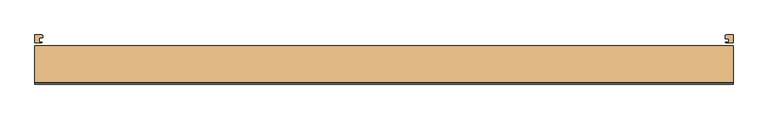
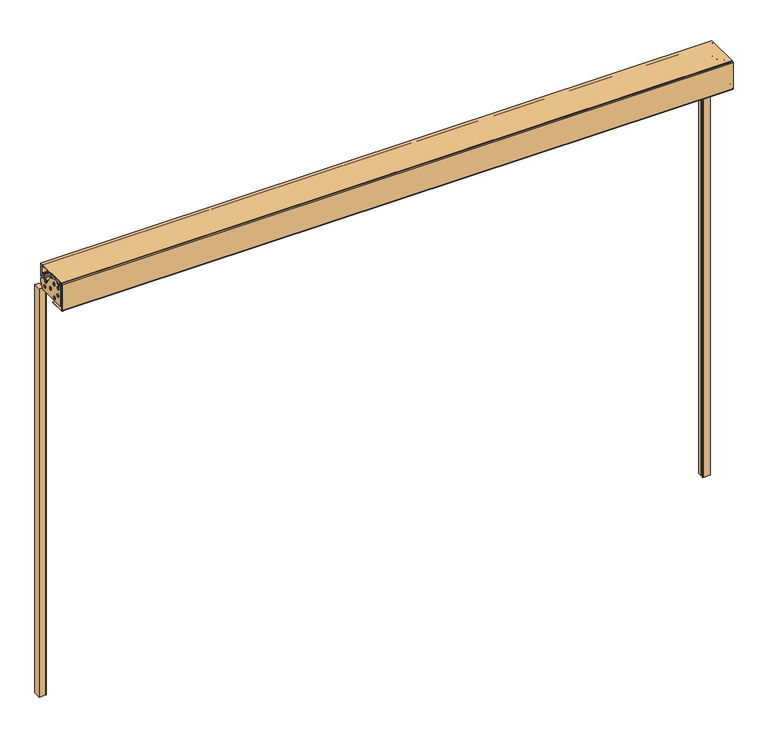
"""IFC4 building model written with IfcOpenShell, lengths in millimetres: door geometry, Otomatik Kapı-Tek Kanat : Otomatik Kapı - Tek Kanat."""

from ifc_helpers import new_model, si_unit, point, frame, frame_2d, origin, origin_with_axes, place, context, project, spatial, polyline, circle_curve, trimmed, segment, composite_curve, outline, extrude, source, transform, mapped, element, save
from ifc_brep_helpers import plane_surface, cylinder_surface, revolved_surface, advanced_brep


def door_4716b48a(model_context):
    return source(origin(), model_context, "Body", "SolidModel", [
        advanced_brep(
        [(1597.0, -299.2542528, 2176.1817261), (1597.0, -285.0832683, 2176.1817261), (1597.0, -280.0474706, 2181.1107692), (1597.0, -280.0474706, 2184.2914876), (1597.0, -239.7553085, 2184.2914876), (1597.0, -239.7553085, 2181.2186799), (1597.0, -234.7183548, 2176.1817261), (1597.0, -226.0109102, 2176.1817261), (1597.0, -221.657188, 2173.7066015), (1597.0, -194.0014824, 2126.1506632), (1597.0, -189.1337497, 2122.4873595), (1597.0, -183.2436236, 2122.4873595), (1597.0, -178.2215661, 2127.509417), (1597.0, -178.2066698, 2136.5727956), (1597.0, -146.96299, 2136.5727956), (1597.0, -146.96299, 2125.3902264), (1597.0, -146.0348324, 2123.5834794), (1597.0, -145.0, 2121.6341872), (1597.0, -145.0, 2108.8285097), (1597.0, -145.5976831, 2106.353385), (1597.0, -161.6461091, 2078.6102552), (1597.0, -165.9998314, 2076.1339745), (1597.0, -299.2542528, 2076.1339745), (1597.0, -304.2900505, 2081.1697722), (1597.0, -304.2900505, 2171.1459284), (1597.0, -252.8153193, 2150.4871347), (1597.0, -252.8153193, 2165.6823884), (1597.0, -286.1075375, 2150.4871347), (1597.0, -286.1075375, 2165.6823884), (1597.0, -284.058999, 2111.9024734), (1597.0, -284.058999, 2126.9266302), (1597.0, -223.621334, 2111.7978536), (1597.0, -223.621334, 2127.0312501), (1597.0, -255.888127, 2083.6460529), (1597.0, -255.888127, 2098.8413066), (1597.0, -176.2436798, 2091.7558144), (1597.0, -176.2436798, 2106.7799712), (1600.0, -299.2542528, 2176.1817261), (1600.0, -304.2900505, 2171.1459284), (1600.0, -304.2900505, 2081.1697722), (1600.0, -299.2542528, 2076.1339745), (1600.0, -165.9998314, 2076.1339745), (1600.0, -161.6461091, 2078.6102552), (1600.0, -145.5976831, 2106.353385), (1600.0, -145.0, 2108.8285097), (1600.0, -145.0, 2121.6341872), (1600.0, -146.0451322, 2123.567749), (1600.0, -146.96299, 2125.3902264), (1600.0, -146.96299, 2136.5727956), (1600.0, -178.2066698, 2136.5727956), (1600.0, -178.2066698, 2127.509417), (1600.0, -183.2436236, 2122.4873595), (1600.0, -189.1337497, 2122.4873595), (1600.0, -194.0014824, 2126.1506632), (1600.0, -221.657188, 2173.7066015), (1600.0, -226.0109102, 2176.1817261), (1600.0, -234.7183548, 2176.1817261), (1600.0, -239.7553085, 2181.2186799), (1600.0, -239.7553085, 2184.2914876), (1600.0, -280.0474706, 2184.2914876), (1600.0, -280.0474706, 2181.1107692), (1600.0, -285.0832683, 2176.1817261), (1600.0, -252.8153193, 2150.4871347), (1600.0, -252.8153193, 2165.6823884), (1600.0, -286.1075375, 2150.4871347), (1600.0, -286.1075375, 2165.6823884), (1600.0, -284.058999, 2111.9024734), (1600.0, -284.058999, 2126.9266302), (1600.0, -223.621334, 2111.7978536), (1600.0, -223.621334, 2127.0312501), (1600.0, -255.888127, 2083.6460529), (1600.0, -255.888127, 2098.8413066), (1600.0, -176.2436798, 2091.7558144), (1600.0, -176.2436798, 2106.7799712)],
        [
            (0, 1),
            (1, 2, circle_curve(frame((1597.0, -285.0832683, 2181.2186799), z_axis=(1.0, 0.0, 0.0), x_axis=(0.0, 0.0, 1.0)), 5.0369538)),
            (2, 3),
            (3, 4),
            (4, 5),
            (5, 6, circle_curve(frame((1597.0, -234.7183548, 2181.2186799), z_axis=(1.0, 0.0, 0.0), x_axis=(0.0, 0.0, 1.0)), 5.0369538)),
            (6, 7),
            (7, 8, circle_curve(frame((1597.0, -225.960249, 2171.2041971), z_axis=(-1.0, 0.0, 0.0), x_axis=(0.0, 0.0, 1.0)), 4.9777868)),
            (8, 9),
            (9, 10, circle_curve(frame((1597.0, -189.1337497, 2127.5530897), z_axis=(1.0, 0.0, 0.0), x_axis=(0.0, 0.0, 1.0)), 5.0657302)),
            (10, 11),
            (11, 12, circle_curve(frame((1597.0, -183.2436236, 2127.509417), z_axis=(1.0, 0.0, 0.0), x_axis=(0.0, 0.0, 1.0)), 5.0220574)),
            (12, 13),
            (13, 14),
            (14, 15),
            (15, 16, circle_curve(frame((1597.0, -144.9082992, 2125.3039782), z_axis=(1.0, 0.0, 0.0), x_axis=(0.0, 0.0, 1.0)), 2.0565002)),
            (16, 17, circle_curve(frame((1597.0, -147.3111729, 2121.6341872), z_axis=(-1.0, 0.0, 0.0), x_axis=(0.0, 0.0, 1.0)), 2.3111729)),
            (17, 18),
            (18, 19, circle_curve(frame((1597.0, -149.4842362, 2108.6016195), z_axis=(-1.0, 0.0, 0.0), x_axis=(0.0, 0.0, 1.0)), 4.4899725)),
            (19, 20),
            (20, 21, circle_curve(frame((1597.0, -165.9399214, 2081.0940748), z_axis=(-1.0, 0.0, 0.0), x_axis=(0.0, 0.0, 1.0)), 4.9604621)),
            (21, 22),
            (22, 23, circle_curve(frame((1597.0, -299.2542528, 2081.1697722), z_axis=(-1.0, 0.0, 0.0), x_axis=(0.0, 0.0, 1.0)), 5.0357977)),
            (23, 24),
            (24, 0, circle_curve(frame((1597.0, -299.2542528, 2171.1459284), z_axis=(-1.0, 0.0, 0.0), x_axis=(0.0, 0.0, 1.0)), 5.0357977)),
            (25, 26, circle_curve(frame((1597.0, -252.8153193, 2158.0847616), z_axis=(1.0, 0.0, 0.0), x_axis=(0.0, 0.0, 1.0)), 7.5976269)),
            (26, 25, circle_curve(frame((1597.0, -252.8153193, 2158.0847616), z_axis=(1.0, 0.0, 0.0), x_axis=(0.0, 0.0, 1.0)), 7.5976269)),
            (27, 28, circle_curve(frame((1597.0, -286.1075375, 2158.0847616), z_axis=(1.0, 0.0, 0.0), x_axis=(0.0, 0.0, 1.0)), 7.5976269)),
            (28, 27, circle_curve(frame((1597.0, -286.1075375, 2158.0847616), z_axis=(1.0, 0.0, 0.0), x_axis=(0.0, 0.0, 1.0)), 7.5976269)),
            (29, 30, circle_curve(frame((1597.0, -284.058999, 2119.4145518), z_axis=(1.0, 0.0, 0.0), x_axis=(0.0, 0.0, 1.0)), 7.5120784)),
            (30, 29, circle_curve(frame((1597.0, -284.058999, 2119.4145518), z_axis=(1.0, 0.0, 0.0), x_axis=(0.0, 0.0, 1.0)), 7.5120784)),
            (31, 32, circle_curve(frame((1597.0, -223.621334, 2119.4145518), z_axis=(1.0, 0.0, 0.0), x_axis=(0.0, 0.0, 1.0)), 7.6166982)),
            (32, 31, circle_curve(frame((1597.0, -223.621334, 2119.4145518), z_axis=(1.0, 0.0, 0.0), x_axis=(0.0, 0.0, 1.0)), 7.6166982)),
            (33, 34, circle_curve(frame((1597.0, -255.888127, 2091.2436798), z_axis=(1.0, 0.0, 0.0), x_axis=(0.0, 0.0, 1.0)), 7.5976269)),
            (34, 33, circle_curve(frame((1597.0, -255.888127, 2091.2436798), z_axis=(1.0, 0.0, 0.0), x_axis=(0.0, 0.0, 1.0)), 7.5976269)),
            (35, 36, circle_curve(frame((1597.0, -176.2436798, 2099.2678928), z_axis=(1.0, 0.0, 0.0), x_axis=(0.0, 0.0, 1.0)), 7.5120784)),
            (36, 35, circle_curve(frame((1597.0, -176.2436798, 2099.2678928), z_axis=(1.0, 0.0, 0.0), x_axis=(0.0, 0.0, 1.0)), 7.5120784)),
            (37, 38, circle_curve(frame((1600.0, -299.2542528, 2171.1459284), z_axis=(1.0, 0.0, 0.0), x_axis=(0.0, 0.0, 1.0)), 5.0357977)),
            (38, 39),
            (39, 40, circle_curve(frame((1600.0, -299.2542528, 2081.1697722), z_axis=(1.0, 0.0, 0.0), x_axis=(0.0, 0.0, 1.0)), 5.0357977)),
            (40, 41),
            (41, 42, circle_curve(frame((1600.0, -165.9399214, 2081.0940748), z_axis=(1.0, 0.0, 0.0), x_axis=(0.0, 0.0, 1.0)), 4.9604621)),
            (42, 43),
            (43, 44, circle_curve(frame((1600.0, -149.4842362, 2108.6016195), z_axis=(1.0, 0.0, 0.0), x_axis=(0.0, 0.0, 1.0)), 4.4899725)),
            (44, 45),
            (45, 46, circle_curve(frame((1600.0, -147.3111729, 2121.6341872), z_axis=(1.0, 0.0, 0.0), x_axis=(0.0, 0.0, 1.0)), 2.3111729)),
            (46, 47, circle_curve(frame((1600.0, -144.9082992, 2125.3039782), z_axis=(-1.0, 0.0, 0.0), x_axis=(0.0, 0.0, 1.0)), 2.0565002)),
            (47, 48),
            (48, 49),
            (49, 50),
            (50, 51, circle_curve(frame((1600.0, -183.2436236, 2127.509417), z_axis=(-1.0, 0.0, 0.0), x_axis=(0.0, 0.0, 1.0)), 5.0220574)),
            (51, 52),
            (52, 53, circle_curve(frame((1600.0, -189.1337497, 2127.5530897), z_axis=(-1.0, 0.0, 0.0), x_axis=(0.0, 0.0, 1.0)), 5.0657302)),
            (53, 54),
            (54, 55, circle_curve(frame((1600.0, -225.960249, 2171.2041971), z_axis=(1.0, 0.0, 0.0), x_axis=(0.0, 0.0, 1.0)), 4.9777868)),
            (55, 56),
            (56, 57, circle_curve(frame((1600.0, -234.7183548, 2181.2186799), z_axis=(-1.0, 0.0, 0.0), x_axis=(0.0, 0.0, 1.0)), 5.0369538)),
            (57, 58),
            (58, 59),
            (59, 60),
            (60, 61, circle_curve(frame((1600.0, -285.0832683, 2181.2186799), z_axis=(-1.0, 0.0, 0.0), x_axis=(0.0, 0.0, 1.0)), 5.0369538)),
            (61, 37),
            (62, 63, circle_curve(frame((1600.0, -252.8153193, 2158.0847616), z_axis=(-1.0, 0.0, 0.0), x_axis=(0.0, 0.0, 1.0)), 7.5976269)),
            (63, 62, circle_curve(frame((1600.0, -252.8153193, 2158.0847616), z_axis=(-1.0, 0.0, 0.0), x_axis=(0.0, 0.0, 1.0)), 7.5976269)),
            (64, 65, circle_curve(frame((1600.0, -286.1075375, 2158.0847616), z_axis=(-1.0, 0.0, 0.0), x_axis=(0.0, 0.0, 1.0)), 7.5976269)),
            (65, 64, circle_curve(frame((1600.0, -286.1075375, 2158.0847616), z_axis=(-1.0, 0.0, 0.0), x_axis=(0.0, 0.0, 1.0)), 7.5976269)),
            (66, 67, circle_curve(frame((1600.0, -284.058999, 2119.4145518), z_axis=(-1.0, 0.0, 0.0), x_axis=(0.0, 0.0, 1.0)), 7.5120784)),
            (67, 66, circle_curve(frame((1600.0, -284.058999, 2119.4145518), z_axis=(-1.0, 0.0, 0.0), x_axis=(0.0, 0.0, 1.0)), 7.5120784)),
            (68, 69, circle_curve(frame((1600.0, -223.621334, 2119.4145518), z_axis=(-1.0, 0.0, 0.0), x_axis=(0.0, 0.0, 1.0)), 7.6166982)),
            (69, 68, circle_curve(frame((1600.0, -223.621334, 2119.4145518), z_axis=(-1.0, 0.0, 0.0), x_axis=(0.0, 0.0, 1.0)), 7.6166982)),
            (70, 71, circle_curve(frame((1600.0, -255.888127, 2091.2436798), z_axis=(-1.0, 0.0, 0.0), x_axis=(0.0, 0.0, 1.0)), 7.5976269)),
            (71, 70, circle_curve(frame((1600.0, -255.888127, 2091.2436798), z_axis=(-1.0, 0.0, 0.0), x_axis=(0.0, 0.0, 1.0)), 7.5976269)),
            (72, 73, circle_curve(frame((1600.0, -176.2436798, 2099.2678928), z_axis=(-1.0, 0.0, 0.0), x_axis=(0.0, 0.0, 1.0)), 7.5120784)),
            (73, 72, circle_curve(frame((1600.0, -176.2436798, 2099.2678928), z_axis=(-1.0, 0.0, 0.0), x_axis=(0.0, 0.0, 1.0)), 7.5120784)),
            (0, 37),
            (61, 1),
            (60, 2),
            (59, 3),
            (58, 4),
            (57, 5),
            (56, 6),
            (55, 7),
            (54, 8),
            (53, 9),
            (52, 10),
            (51, 11),
            (50, 12),
            (49, 13),
            (48, 14),
            (47, 15),
            (46, 16),
            (45, 17),
            (44, 18),
            (43, 19),
            (42, 20),
            (41, 21),
            (40, 22),
            (39, 23),
            (38, 24),
            (25, 62),
            (63, 26),
            (27, 64),
            (65, 28),
            (29, 66),
            (67, 30),
            (31, 68),
            (69, 32),
            (33, 70),
            (71, 34),
            (35, 72),
            (73, 36),
        ],
        [
            plane_surface(frame((1597.0, -145.0, 2060.0), z_axis=(-1.0, 0.0, 0.0), x_axis=(0.0, -1.0, 0.0))),
            plane_surface(frame((1600.0, -145.0, 2060.0), z_axis=(1.0, 0.0, 0.0), x_axis=(0.0, -1.0, 0.0))),
            plane_surface(frame((1597.0, -299.2542528, 2176.1817261), z_axis=(0.0, 0.0, 1.0), x_axis=(1.0, 0.0, 0.0))),
            revolved_surface(polyline([(1600.0, -285.0832683, 2186.2556337), (1597.0, -285.0832683, 2186.2556337)]), (1597.0, -285.0832683, 2181.2186799), (1.0, 0.0, 0.0)),
            plane_surface(frame((1597.0, -280.0474706, 2181.1107692), z_axis=(0.0, -1.0, 0.0), x_axis=(1.0, 0.0, 0.0))),
            plane_surface(frame((1597.0, -280.0474706, 2184.2914876), z_axis=(0.0, 0.0, 1.0), x_axis=(1.0, 0.0, 0.0))),
            plane_surface(frame((1597.0, -239.7553085, 2184.2914876), z_axis=(0.0, 1.0, 0.0), x_axis=(1.0, 0.0, 0.0))),
            revolved_surface(polyline([(1600.0, -234.7183548, 2186.2556337), (1597.0, -234.7183548, 2186.2556337)]), (1597.0, -234.7183548, 2181.2186799), (1.0, 0.0, 0.0)),
            plane_surface(frame((1597.0, -234.7183548, 2176.1817261), z_axis=(0.0, 0.0, 1.0), x_axis=(1.0, 0.0, 0.0))),
            cylinder_surface(frame((1597.0, -225.960249, 2171.2041971), z_axis=(-1.0, 0.0, 0.0), x_axis=(0.0, 0.0, 1.0)), 4.9777868),
            plane_surface(frame((1597.0, -221.657188, 2173.7066015), z_axis=(0.0, 0.8644526484288484, 0.5027142514633436), x_axis=(1.0, 0.0, 0.0))),
            revolved_surface(polyline([(1600.0, -189.1337497, 2132.6188199), (1597.0, -189.1337497, 2132.6188199)]), (1597.0, -189.1337497, 2127.5530897), (1.0, 0.0, 0.0)),
            plane_surface(frame((1597.0, -189.1337497, 2122.4873595), z_axis=(0.0, 0.0, 1.0), x_axis=(1.0, 0.0, 0.0))),
            revolved_surface(polyline([(1600.0, -183.2436236, 2132.5314744), (1597.0, -183.2436236, 2132.5314744)]), (1597.0, -183.2436236, 2127.509417), (1.0, 0.0, 0.0)),
            plane_surface(frame((1597.0, -178.2066698, 2127.509417), z_axis=(0.0, -1.0, 0.0), x_axis=(1.0, 0.0, 0.0))),
            plane_surface(frame((1597.0, -178.2066698, 2136.5727956), z_axis=(0.0, 0.0, 1.0), x_axis=(1.0, 0.0, 0.0))),
            plane_surface(frame((1597.0, -146.96299, 2136.5727956), z_axis=(0.0, 1.0, 0.0), x_axis=(1.0, 0.0, 0.0))),
            revolved_surface(polyline([(1600.0, -144.9082992, 2127.3604784), (1597.0, -144.9082992, 2127.3604784)]), (1597.0, -144.9082992, 2125.3039782), (1.0, 0.0, 0.0)),
            cylinder_surface(frame((1597.0, -147.3111729, 2121.6341872), z_axis=(-1.0, 0.0, 0.0), x_axis=(0.0, 0.0, 1.0)), 2.3111729),
            plane_surface(frame((1597.0, -145.0, 2121.6341872), z_axis=(0.0, 1.0, 0.0), x_axis=(1.0, 0.0, 0.0))),
            cylinder_surface(frame((1597.0, -149.4842362, 2108.6016195), z_axis=(-1.0, 0.0, 0.0), x_axis=(0.0, 0.0, 1.0)), 4.4899725),
            plane_surface(frame((1597.0, -145.5976831, 2106.353385), z_axis=(0.0, 0.8656073271784467, -0.5007234317814432), x_axis=(1.0, 0.0, 0.0))),
            cylinder_surface(frame((1597.0, -165.9399214, 2081.0940748), z_axis=(-1.0, 0.0, 0.0), x_axis=(0.0, 0.0, 1.0)), 4.9604621),
            plane_surface(frame((1597.0, -165.9998314, 2076.1339745), z_axis=(0.0, 0.0, -1.0), x_axis=(1.0, 0.0, 0.0))),
            cylinder_surface(frame((1597.0, -299.2542528, 2081.1697722), z_axis=(-1.0, 0.0, 0.0), x_axis=(0.0, 0.0, 1.0)), 5.0357977),
            plane_surface(frame((1597.0, -304.2900505, 2081.1697722), z_axis=(0.0, -1.0, 0.0), x_axis=(1.0, 0.0, 0.0))),
            cylinder_surface(frame((1597.0, -299.2542528, 2171.1459284), z_axis=(-1.0, 0.0, 0.0), x_axis=(0.0, 0.0, 1.0)), 5.0357977),
            revolved_surface(polyline([(1600.0, -252.8153193, 2165.6823885), (1597.0, -252.8153193, 2165.6823885)]), (1597.0, -252.8153193, 2158.0847616), (1.0, 0.0, 0.0)),
            revolved_surface(polyline([(1600.0, -286.1075375, 2165.6823885), (1597.0, -286.1075375, 2165.6823885)]), (1597.0, -286.1075375, 2158.0847616), (1.0, 0.0, 0.0)),
            revolved_surface(polyline([(1600.0, -284.058999, 2126.9266302), (1597.0, -284.058999, 2126.9266302)]), (1597.0, -284.058999, 2119.4145518), (1.0, 0.0, 0.0)),
            revolved_surface(polyline([(1600.0, -223.621334, 2127.03125), (1597.0, -223.621334, 2127.03125)]), (1597.0, -223.621334, 2119.4145518), (1.0, 0.0, 0.0)),
            revolved_surface(polyline([(1600.0, -255.888127, 2098.8413066999997), (1597.0, -255.888127, 2098.8413066999997)]), (1597.0, -255.888127, 2091.2436798), (1.0, 0.0, 0.0)),
            revolved_surface(polyline([(1600.0, -176.2436798, 2106.7799712), (1597.0, -176.2436798, 2106.7799712)]), (1597.0, -176.2436798, 2099.2678928), (1.0, 0.0, 0.0)),
        ],
        [
            (0, [[1, 2, 3, 4, 5, 6, 7, 8, 9, 10, 11, 12, 13, 14, 15, 16, 17, 18, 19, 20, 21, 22, 23, 24, 25], [26, 27], [28, 29], [30, 31], [32, 33], [34, 35], [36, 37]]),
            (1, [[38, 39, 40, 41, 42, 43, 44, 45, 46, 47, 48, 49, 50, 51, 52, 53, 54, 55, 56, 57, 58, 59, 60, 61, 62], [63, 64], [65, 66], [67, 68], [69, 70], [71, 72], [73, 74]]),
            (2, [[-1, 75, -62, 76]]),
            (3, [[-2, -76, -61, 77]]),
            (4, [[-3, -77, -60, 78]]),
            (5, [[-4, -78, -59, 79]]),
            (6, [[-5, -79, -58, 80]]),
            (7, [[-6, -80, -57, 81]]),
            (8, [[-7, -81, -56, 82]]),
            (9, [[-8, -82, -55, 83]]),
            (10, [[-9, -83, -54, 84]]),
            (11, [[-10, -84, -53, 85]]),
            (12, [[-11, -85, -52, 86]]),
            (13, [[-12, -86, -51, 87]]),
            (14, [[-13, -87, -50, 88]]),
            (15, [[-14, -88, -49, 89]]),
            (16, [[-15, -89, -48, 90]]),
            (17, [[-16, -90, -47, 91]]),
            (18, [[-17, -91, -46, 92]]),
            (19, [[-18, -92, -45, 93]]),
            (20, [[-19, -93, -44, 94]]),
            (21, [[-20, -94, -43, 95]]),
            (22, [[-21, -95, -42, 96]]),
            (23, [[-22, -96, -41, 97]]),
            (24, [[-23, -97, -40, 98]]),
            (25, [[-24, -98, -39, 99]]),
            (26, [[-25, -99, -38, -75]]),
            (27, [[-26, 100, -64, 101]]),
            (27, [[-27, -101, -63, -100]]),
            (28, [[-28, 102, -66, 103]]),
            (28, [[-29, -103, -65, -102]]),
            (29, [[-30, 104, -68, 105]]),
            (29, [[-31, -105, -67, -104]]),
            (30, [[-32, 106, -70, 107]]),
            (30, [[-33, -107, -69, -106]]),
            (31, [[-34, 108, -72, 109]]),
            (31, [[-35, -109, -71, -108]]),
            (32, [[-36, 110, -74, 111]]),
            (32, [[-37, -111, -73, -110]]),
        ],
    ),
        advanced_brep(
        [(-1597.0, -239.7553085, 2184.2914876), (-1597.0, -280.0474706, 2184.2914876), (-1597.0, -280.0474706, 2181.1107692), (-1597.0, -285.0832683, 2176.1817261), (-1597.0, -299.2542528, 2176.1817261), (-1597.0, -304.2900505, 2171.1459284), (-1597.0, -304.2900505, 2081.1697722), (-1597.0, -299.2542528, 2076.1339745), (-1597.0, -165.9998314, 2076.1339745), (-1597.0, -161.6461091, 2078.6102552), (-1597.0, -145.5976831, 2106.353385), (-1597.0, -145.0, 2108.8285097), (-1597.0, -145.0, 2121.6341872), (-1597.0, -146.0451322, 2123.567749), (-1597.0, -146.96299, 2125.3902264), (-1597.0, -146.96299, 2136.5727956), (-1597.0, -178.2066698, 2136.5727956), (-1597.0, -178.2066698, 2127.509417), (-1597.0, -183.2436236, 2122.4873595), (-1597.0, -189.1337497, 2122.4873595), (-1597.0, -194.0014824, 2126.1506632), (-1597.0, -221.657188, 2173.7066015), (-1597.0, -226.0109102, 2176.1817261), (-1597.0, -234.7183548, 2176.1817261), (-1597.0, -239.7553085, 2181.2186799), (-1597.0, -176.2436798, 2106.7799712), (-1597.0, -176.2436798, 2091.7558144), (-1597.0, -223.621334, 2127.0312501), (-1597.0, -223.621334, 2111.7978536), (-1597.0, -252.8153193, 2165.6823884), (-1597.0, -252.8153193, 2150.4871347), (-1597.0, -286.1075375, 2165.6823884), (-1597.0, -286.1075375, 2150.4871347), (-1597.0, -284.058999, 2126.9266302), (-1597.0, -284.058999, 2111.9024734), (-1597.0, -255.888127, 2098.8413066), (-1597.0, -255.888127, 2083.6460529), (-1600.0, -239.7553085, 2184.2914876), (-1600.0, -239.7553085, 2181.2186799), (-1600.0, -234.7183548, 2176.1817261), (-1600.0, -226.0109102, 2176.1817261), (-1600.0, -221.657188, 2173.7066015), (-1600.0, -194.0014824, 2126.1506632), (-1600.0, -189.1337497, 2122.4873595), (-1600.0, -183.2436236, 2122.4873595), (-1600.0, -178.2215661, 2127.509417), (-1600.0, -178.2066698, 2136.5727956), (-1600.0, -146.96299, 2136.5727956), (-1600.0, -146.96299, 2125.3902264), (-1600.0, -146.0348324, 2123.5834794), (-1600.0, -145.0, 2121.6341872), (-1600.0, -145.0, 2108.8285097), (-1600.0, -145.5976831, 2106.353385), (-1600.0, -161.6461091, 2078.6102552), (-1600.0, -165.9998314, 2076.1339745), (-1600.0, -299.2542528, 2076.1339745), (-1600.0, -304.2900505, 2081.1697722), (-1600.0, -304.2900505, 2171.1459284), (-1600.0, -299.2542528, 2176.1817261), (-1600.0, -285.0832683, 2176.1817261), (-1600.0, -280.0474706, 2181.1107692), (-1600.0, -280.0474706, 2184.2914876), (-1600.0, -176.2436798, 2106.7799712), (-1600.0, -176.2436798, 2091.7558144), (-1600.0, -223.621334, 2127.0312501), (-1600.0, -223.621334, 2111.7978536), (-1600.0, -252.8153193, 2165.6823884), (-1600.0, -252.8153193, 2150.4871347), (-1600.0, -286.1075375, 2165.6823884), (-1600.0, -286.1075375, 2150.4871347), (-1600.0, -284.058999, 2126.9266302), (-1600.0, -284.058999, 2111.9024734), (-1600.0, -255.888127, 2098.8413066), (-1600.0, -255.888127, 2083.6460529)],
        [
            (0, 1),
            (1, 2),
            (2, 3, circle_curve(frame((-1597.0, -285.0832683, 2181.2186799), z_axis=(-1.0, 0.0, 0.0), x_axis=(0.0, 0.0, -1.0)), 5.0369538)),
            (3, 4),
            (4, 5, circle_curve(frame((-1597.0, -299.2542528, 2171.1459284), z_axis=(1.0, 0.0, 0.0), x_axis=(0.0, 0.0, -1.0)), 5.0357977)),
            (5, 6),
            (6, 7, circle_curve(frame((-1597.0, -299.2542528, 2081.1697722), z_axis=(1.0, 0.0, 0.0), x_axis=(0.0, 0.0, -1.0)), 5.0357977)),
            (7, 8),
            (8, 9, circle_curve(frame((-1597.0, -165.9399214, 2081.0940748), z_axis=(1.0, 0.0, 0.0), x_axis=(0.0, 0.0, -1.0)), 4.9604621)),
            (9, 10),
            (10, 11, circle_curve(frame((-1597.0, -149.4842362, 2108.6016195), z_axis=(1.0, 0.0, 0.0), x_axis=(0.0, 0.0, -1.0)), 4.4899725)),
            (11, 12),
            (12, 13, circle_curve(frame((-1597.0, -147.3111729, 2121.6341872), z_axis=(1.0, 0.0, 0.0), x_axis=(0.0, 0.0, -1.0)), 2.3111729)),
            (13, 14, circle_curve(frame((-1597.0, -144.9082992, 2125.3039782), z_axis=(-1.0, 0.0, 0.0), x_axis=(0.0, 0.0, -1.0)), 2.0565002)),
            (14, 15),
            (15, 16),
            (16, 17),
            (17, 18, circle_curve(frame((-1597.0, -183.2436236, 2127.509417), z_axis=(-1.0, 0.0, 0.0), x_axis=(0.0, 0.0, -1.0)), 5.0220574)),
            (18, 19),
            (19, 20, circle_curve(frame((-1597.0, -189.1337497, 2127.5530897), z_axis=(-1.0, 0.0, 0.0), x_axis=(0.0, 0.0, -1.0)), 5.0657302)),
            (20, 21),
            (21, 22, circle_curve(frame((-1597.0, -225.960249, 2171.2041971), z_axis=(1.0, 0.0, 0.0), x_axis=(0.0, 0.0, -1.0)), 4.9777868)),
            (22, 23),
            (23, 24, circle_curve(frame((-1597.0, -234.7183548, 2181.2186799), z_axis=(-1.0, 0.0, 0.0), x_axis=(0.0, 0.0, -1.0)), 5.0369538)),
            (24, 0),
            (25, 26, circle_curve(frame((-1597.0, -176.2436798, 2099.2678928), z_axis=(-1.0, 0.0, 0.0), x_axis=(0.0, 0.0, -1.0)), 7.5120784)),
            (26, 25, circle_curve(frame((-1597.0, -176.2436798, 2099.2678928), z_axis=(-1.0, 0.0, 0.0), x_axis=(0.0, 0.0, -1.0)), 7.5120784)),
            (27, 28, circle_curve(frame((-1597.0, -223.621334, 2119.4145518), z_axis=(-1.0, 0.0, 0.0), x_axis=(0.0, 0.0, -1.0)), 7.6166982)),
            (28, 27, circle_curve(frame((-1597.0, -223.621334, 2119.4145518), z_axis=(-1.0, 0.0, 0.0), x_axis=(0.0, 0.0, -1.0)), 7.6166982)),
            (29, 30, circle_curve(frame((-1597.0, -252.8153193, 2158.0847616), z_axis=(-1.0, 0.0, 0.0), x_axis=(0.0, 0.0, -1.0)), 7.5976269)),
            (30, 29, circle_curve(frame((-1597.0, -252.8153193, 2158.0847616), z_axis=(-1.0, 0.0, 0.0), x_axis=(0.0, 0.0, -1.0)), 7.5976269)),
            (31, 32, circle_curve(frame((-1597.0, -286.1075375, 2158.0847616), z_axis=(-1.0, 0.0, 0.0), x_axis=(0.0, 0.0, -1.0)), 7.5976269)),
            (32, 31, circle_curve(frame((-1597.0, -286.1075375, 2158.0847616), z_axis=(-1.0, 0.0, 0.0), x_axis=(0.0, 0.0, -1.0)), 7.5976269)),
            (33, 34, circle_curve(frame((-1597.0, -284.058999, 2119.4145518), z_axis=(-1.0, 0.0, 0.0), x_axis=(0.0, 0.0, -1.0)), 7.5120784)),
            (34, 33, circle_curve(frame((-1597.0, -284.058999, 2119.4145518), z_axis=(-1.0, 0.0, 0.0), x_axis=(0.0, 0.0, -1.0)), 7.5120784)),
            (35, 36, circle_curve(frame((-1597.0, -255.888127, 2091.2436798), z_axis=(-1.0, 0.0, 0.0), x_axis=(0.0, 0.0, -1.0)), 7.5976269)),
            (36, 35, circle_curve(frame((-1597.0, -255.888127, 2091.2436798), z_axis=(-1.0, 0.0, 0.0), x_axis=(0.0, 0.0, -1.0)), 7.5976269)),
            (37, 38),
            (38, 39, circle_curve(frame((-1600.0, -234.7183548, 2181.2186799), z_axis=(1.0, 0.0, 0.0), x_axis=(0.0, 0.0, -1.0)), 5.0369538)),
            (39, 40),
            (40, 41, circle_curve(frame((-1600.0, -225.960249, 2171.2041971), z_axis=(-1.0, 0.0, 0.0), x_axis=(0.0, 0.0, -1.0)), 4.9777868)),
            (41, 42),
            (42, 43, circle_curve(frame((-1600.0, -189.1337497, 2127.5530897), z_axis=(1.0, 0.0, 0.0), x_axis=(0.0, 0.0, -1.0)), 5.0657302)),
            (43, 44),
            (44, 45, circle_curve(frame((-1600.0, -183.2436236, 2127.509417), z_axis=(1.0, 0.0, 0.0), x_axis=(0.0, 0.0, -1.0)), 5.0220574)),
            (45, 46),
            (46, 47),
            (47, 48),
            (48, 49, circle_curve(frame((-1600.0, -144.9082992, 2125.3039782), z_axis=(1.0, 0.0, 0.0), x_axis=(0.0, 0.0, -1.0)), 2.0565002)),
            (49, 50, circle_curve(frame((-1600.0, -147.3111729, 2121.6341872), z_axis=(-1.0, 0.0, 0.0), x_axis=(0.0, 0.0, -1.0)), 2.3111729)),
            (50, 51),
            (51, 52, circle_curve(frame((-1600.0, -149.4842362, 2108.6016195), z_axis=(-1.0, 0.0, 0.0), x_axis=(0.0, 0.0, -1.0)), 4.4899725)),
            (52, 53),
            (53, 54, circle_curve(frame((-1600.0, -165.9399214, 2081.0940748), z_axis=(-1.0, 0.0, 0.0), x_axis=(0.0, 0.0, -1.0)), 4.9604621)),
            (54, 55),
            (55, 56, circle_curve(frame((-1600.0, -299.2542528, 2081.1697722), z_axis=(-1.0, 0.0, 0.0), x_axis=(0.0, 0.0, -1.0)), 5.0357977)),
            (56, 57),
            (57, 58, circle_curve(frame((-1600.0, -299.2542528, 2171.1459284), z_axis=(-1.0, 0.0, 0.0), x_axis=(0.0, 0.0, -1.0)), 5.0357977)),
            (58, 59),
            (59, 60, circle_curve(frame((-1600.0, -285.0832683, 2181.2186799), z_axis=(1.0, 0.0, 0.0), x_axis=(0.0, 0.0, -1.0)), 5.0369538)),
            (60, 61),
            (61, 37),
            (62, 63, circle_curve(frame((-1600.0, -176.2436798, 2099.2678928), z_axis=(1.0, 0.0, 0.0), x_axis=(0.0, 0.0, -1.0)), 7.5120784)),
            (63, 62, circle_curve(frame((-1600.0, -176.2436798, 2099.2678928), z_axis=(1.0, 0.0, 0.0), x_axis=(0.0, 0.0, -1.0)), 7.5120784)),
            (64, 65, circle_curve(frame((-1600.0, -223.621334, 2119.4145518), z_axis=(1.0, 0.0, 0.0), x_axis=(0.0, 0.0, -1.0)), 7.6166982)),
            (65, 64, circle_curve(frame((-1600.0, -223.621334, 2119.4145518), z_axis=(1.0, 0.0, 0.0), x_axis=(0.0, 0.0, -1.0)), 7.6166982)),
            (66, 67, circle_curve(frame((-1600.0, -252.8153193, 2158.0847616), z_axis=(1.0, 0.0, 0.0), x_axis=(0.0, 0.0, -1.0)), 7.5976269)),
            (67, 66, circle_curve(frame((-1600.0, -252.8153193, 2158.0847616), z_axis=(1.0, 0.0, 0.0), x_axis=(0.0, 0.0, -1.0)), 7.5976269)),
            (68, 69, circle_curve(frame((-1600.0, -286.1075375, 2158.0847616), z_axis=(1.0, 0.0, 0.0), x_axis=(0.0, 0.0, -1.0)), 7.5976269)),
            (69, 68, circle_curve(frame((-1600.0, -286.1075375, 2158.0847616), z_axis=(1.0, 0.0, 0.0), x_axis=(0.0, 0.0, -1.0)), 7.5976269)),
            (70, 71, circle_curve(frame((-1600.0, -284.058999, 2119.4145518), z_axis=(1.0, 0.0, 0.0), x_axis=(0.0, 0.0, -1.0)), 7.5120784)),
            (71, 70, circle_curve(frame((-1600.0, -284.058999, 2119.4145518), z_axis=(1.0, 0.0, 0.0), x_axis=(0.0, 0.0, -1.0)), 7.5120784)),
            (72, 73, circle_curve(frame((-1600.0, -255.888127, 2091.2436798), z_axis=(1.0, 0.0, 0.0), x_axis=(0.0, 0.0, -1.0)), 7.5976269)),
            (73, 72, circle_curve(frame((-1600.0, -255.888127, 2091.2436798), z_axis=(1.0, 0.0, 0.0), x_axis=(0.0, 0.0, -1.0)), 7.5976269)),
            (0, 37),
            (61, 1),
            (60, 2),
            (59, 3),
            (58, 4),
            (57, 5),
            (56, 6),
            (55, 7),
            (54, 8),
            (53, 9),
            (52, 10),
            (51, 11),
            (50, 12),
            (49, 13),
            (48, 14),
            (47, 15),
            (46, 16),
            (45, 17),
            (44, 18),
            (43, 19),
            (42, 20),
            (41, 21),
            (40, 22),
            (39, 23),
            (38, 24),
            (25, 62),
            (63, 26),
            (27, 64),
            (65, 28),
            (29, 66),
            (67, 30),
            (31, 68),
            (69, 32),
            (33, 70),
            (71, 34),
            (35, 72),
            (73, 36),
        ],
        [
            plane_surface(frame((-1597.0, -145.0, 2059.9969475), z_axis=(1.0, 0.0, 0.0), x_axis=(0.0, -1.0, 0.0))),
            plane_surface(frame((-1600.0, -145.0, 2059.9969475), z_axis=(-1.0, 0.0, 0.0), x_axis=(0.0, -1.0, 0.0))),
            plane_surface(frame((-1597.0, -239.7553085, 2184.2914876), z_axis=(0.0, 0.0, 1.0), x_axis=(-1.0, 0.0, 0.0))),
            plane_surface(frame((-1597.0, -280.0474706, 2184.2914876), z_axis=(0.0, -1.0, 0.0), x_axis=(-1.0, 0.0, 0.0))),
            revolved_surface(polyline([(-1600.0, -285.0832683, 2176.1817261), (-1597.0, -285.0832683, 2176.1817261)]), (-1597.0, -285.0832683, 2181.2186799), (-1.0, 0.0, 0.0)),
            plane_surface(frame((-1597.0, -285.0832683, 2176.1817261), z_axis=(0.0, 0.0, 1.0), x_axis=(-1.0, 0.0, 0.0))),
            cylinder_surface(frame((-1597.0, -299.2542528, 2171.1459284), z_axis=(1.0, 0.0, 0.0), x_axis=(0.0, 0.0, -1.0)), 5.0357977),
            plane_surface(frame((-1597.0, -304.2900505, 2171.1459284), z_axis=(0.0, -1.0, 0.0), x_axis=(-1.0, 0.0, 0.0))),
            cylinder_surface(frame((-1597.0, -299.2542528, 2081.1697722), z_axis=(1.0, 0.0, 0.0), x_axis=(0.0, 0.0, -1.0)), 5.0357977),
            plane_surface(frame((-1597.0, -299.2542528, 2076.1339745), z_axis=(0.0, 0.0, -1.0), x_axis=(-1.0, 0.0, 0.0))),
            cylinder_surface(frame((-1597.0, -165.9399214, 2081.0940748), z_axis=(1.0, 0.0, 0.0), x_axis=(0.0, 0.0, -1.0)), 4.9604621),
            plane_surface(frame((-1597.0, -161.6461091, 2078.6102552), z_axis=(0.0, 0.8656073271784469, -0.5007234317814427), x_axis=(-1.0, 0.0, 0.0))),
            cylinder_surface(frame((-1597.0, -149.4842362, 2108.6016195), z_axis=(1.0, 0.0, 0.0), x_axis=(0.0, 0.0, -1.0)), 4.4899725),
            plane_surface(frame((-1597.0, -145.0, 2108.8285097), z_axis=(0.0, 1.0, 0.0), x_axis=(-1.0, 0.0, 0.0))),
            cylinder_surface(frame((-1597.0, -147.3111729, 2121.6341872), z_axis=(1.0, 0.0, 0.0), x_axis=(0.0, 0.0, -1.0)), 2.3111729),
            revolved_surface(polyline([(-1600.0, -144.9082992, 2123.2474780000002), (-1597.0, -144.9082992, 2123.2474780000002)]), (-1597.0, -144.9082992, 2125.3039782), (-1.0, 0.0, 0.0)),
            plane_surface(frame((-1597.0, -146.96299, 2125.3902264), z_axis=(0.0, 1.0, 0.0), x_axis=(-1.0, 0.0, 0.0))),
            plane_surface(frame((-1597.0, -146.96299, 2136.5727956), z_axis=(0.0, 0.0, 1.0), x_axis=(-1.0, 0.0, 0.0))),
            plane_surface(frame((-1597.0, -178.2066698, 2136.5727956), z_axis=(0.0, -1.0, 0.0), x_axis=(-1.0, 0.0, 0.0))),
            revolved_surface(polyline([(-1600.0, -183.2436236, 2122.4873596), (-1597.0, -183.2436236, 2122.4873596)]), (-1597.0, -183.2436236, 2127.509417), (-1.0, 0.0, 0.0)),
            plane_surface(frame((-1597.0, -183.2436236, 2122.4873595), z_axis=(0.0, 0.0, 1.0), x_axis=(-1.0, 0.0, 0.0))),
            revolved_surface(polyline([(-1600.0, -189.1337497, 2122.4873595), (-1597.0, -189.1337497, 2122.4873595)]), (-1597.0, -189.1337497, 2127.5530897), (-1.0, 0.0, 0.0)),
            plane_surface(frame((-1597.0, -194.0014824, 2126.1506632), z_axis=(0.0, 0.8644526484288326, 0.5027142514633708), x_axis=(-1.0, 0.0, 0.0))),
            cylinder_surface(frame((-1597.0, -225.960249, 2171.2041971), z_axis=(1.0, 0.0, 0.0), x_axis=(0.0, 0.0, -1.0)), 4.9777868),
            plane_surface(frame((-1597.0, -226.0109102, 2176.1817261), z_axis=(0.0, 0.0, 1.0), x_axis=(-1.0, 0.0, 0.0))),
            revolved_surface(polyline([(-1600.0, -234.7183548, 2176.1817261), (-1597.0, -234.7183548, 2176.1817261)]), (-1597.0, -234.7183548, 2181.2186799), (-1.0, 0.0, 0.0)),
            plane_surface(frame((-1597.0, -239.7553085, 2181.2186799), z_axis=(0.0, 1.0, 0.0), x_axis=(-1.0, 0.0, 0.0))),
            revolved_surface(polyline([(-1600.0, -176.2436798, 2091.7558144), (-1597.0, -176.2436798, 2091.7558144)]), (-1597.0, -176.2436798, 2099.2678928), (-1.0, 0.0, 0.0)),
            revolved_surface(polyline([(-1600.0, -223.621334, 2111.7978536), (-1597.0, -223.621334, 2111.7978536)]), (-1597.0, -223.621334, 2119.4145518), (-1.0, 0.0, 0.0)),
            revolved_surface(polyline([(-1600.0, -252.8153193, 2150.4871347000003), (-1597.0, -252.8153193, 2150.4871347000003)]), (-1597.0, -252.8153193, 2158.0847616), (-1.0, 0.0, 0.0)),
            revolved_surface(polyline([(-1600.0, -286.1075375, 2150.4871347000003), (-1597.0, -286.1075375, 2150.4871347000003)]), (-1597.0, -286.1075375, 2158.0847616), (-1.0, 0.0, 0.0)),
            revolved_surface(polyline([(-1600.0, -284.058999, 2111.9024734), (-1597.0, -284.058999, 2111.9024734)]), (-1597.0, -284.058999, 2119.4145518), (-1.0, 0.0, 0.0)),
            revolved_surface(polyline([(-1600.0, -255.888127, 2083.6460529), (-1597.0, -255.888127, 2083.6460529)]), (-1597.0, -255.888127, 2091.2436798), (-1.0, 0.0, 0.0)),
        ],
        [
            (0, [[1, 2, 3, 4, 5, 6, 7, 8, 9, 10, 11, 12, 13, 14, 15, 16, 17, 18, 19, 20, 21, 22, 23, 24, 25], [26, 27], [28, 29], [30, 31], [32, 33], [34, 35], [36, 37]]),
            (1, [[38, 39, 40, 41, 42, 43, 44, 45, 46, 47, 48, 49, 50, 51, 52, 53, 54, 55, 56, 57, 58, 59, 60, 61, 62], [63, 64], [65, 66], [67, 68], [69, 70], [71, 72], [73, 74]]),
            (2, [[-1, 75, -62, 76]]),
            (3, [[-2, -76, -61, 77]]),
            (4, [[-3, -77, -60, 78]]),
            (5, [[-4, -78, -59, 79]]),
            (6, [[-5, -79, -58, 80]]),
            (7, [[-6, -80, -57, 81]]),
            (8, [[-7, -81, -56, 82]]),
            (9, [[-8, -82, -55, 83]]),
            (10, [[-9, -83, -54, 84]]),
            (11, [[-10, -84, -53, 85]]),
            (12, [[-11, -85, -52, 86]]),
            (13, [[-12, -86, -51, 87]]),
            (14, [[-13, -87, -50, 88]]),
            (15, [[-14, -88, -49, 89]]),
            (16, [[-15, -89, -48, 90]]),
            (17, [[-16, -90, -47, 91]]),
            (18, [[-17, -91, -46, 92]]),
            (19, [[-18, -92, -45, 93]]),
            (20, [[-19, -93, -44, 94]]),
            (21, [[-20, -94, -43, 95]]),
            (22, [[-21, -95, -42, 96]]),
            (23, [[-22, -96, -41, 97]]),
            (24, [[-23, -97, -40, 98]]),
            (25, [[-24, -98, -39, 99]]),
            (26, [[-25, -99, -38, -75]]),
            (27, [[-26, 100, -64, 101]]),
            (27, [[-27, -101, -63, -100]]),
            (28, [[-28, 102, -66, 103]]),
            (28, [[-29, -103, -65, -102]]),
            (29, [[-30, 104, -68, 105]]),
            (29, [[-31, -105, -67, -104]]),
            (30, [[-32, 106, -70, 107]]),
            (30, [[-33, -107, -69, -106]]),
            (31, [[-34, 108, -72, 109]]),
            (31, [[-35, -109, -71, -108]]),
            (32, [[-36, 110, -74, 111]]),
            (32, [[-37, -111, -73, -110]]),
        ],
    ),
        extrude(outline(composite_curve([segment(polyline([(-311.5000025, 2200.0002021), (-145.0, 2199.9997337), (-145.0, 2135.9993507), (-146.4999995, 2135.9993507), (-146.5000017, 2144.1994972)]), True, "CONTINUOUS"), segment(trimmed(circle_curve(frame_2d((-147.5000017, 2144.1994972)), 1.0), [point((-146.5000017, 2144.1994972))], [point((-147.5000004, 2145.1994972))], True, "CARTESIAN"), True, "CONTINUOUS"), segment(polyline([(-147.5000004, 2145.1994972), (-158.5000018, 2145.1995108), (-158.5000005, 2139.9993507), (-169.3003272, 2139.9993507), (-169.3003272, 2137.9993047), (-172.7003364, 2137.9993047), (-172.7003398, 2135.9993045), (-192.0003011, 2135.9993507)]), True, "CONTINUOUS"), segment(trimmed(circle_curve(frame_2d((-192.0003011, 2137.9993508)), 2.0), [point((-192.0003011, 2135.9993507))], [point((-194.0003011, 2137.9993508))], False, "CARTESIAN"), True, "CONTINUOUS"), segment(polyline([(-194.0003011, 2137.9993508), (-194.0003011, 2141.7851316)]), True, "CONTINUOUS"), segment(trimmed(circle_curve(frame_2d((-184.9754732, 2122.7091902)), 21.1030581), [point((-194.0003011, 2141.7851316))], [point((-176.1755405, 2141.8899161))], False, "CARTESIAN"), True, "CONTINUOUS"), segment(polyline([(-176.1755405, 2141.8899161), (-175.7006399, 2141.249351), (-174.7003519, 2141.249351)]), True, "CONTINUOUS"), segment(trimmed(circle_curve(frame_2d((-174.7003519, 2142.2493509)), 1.0), [point((-174.7003519, 2141.249351))], [point((-173.7003519, 2142.2493509))], True, "CARTESIAN"), True, "CONTINUOUS"), segment(polyline([(-173.7003519, 2142.2493509), (-173.7003519, 2147.7993514)]), True, "CONTINUOUS"), segment(trimmed(circle_curve(frame_2d((-168.7003517, 2147.7993512)), 5.0), [point((-173.7003519, 2147.7993514))], [point((-168.7003517, 2152.7993512))], False, "CARTESIAN"), True, "CONTINUOUS"), segment(polyline([(-168.7003517, 2152.7993512), (-165.5837187, 2152.7993512), (-155.8803848, 2150.1993508), (-152.0, 2150.1993508)]), True, "CONTINUOUS"), segment(trimmed(circle_curve(frame_2d((-152.0, 2152.1993508)), 2.0), [point((-152.0, 2150.1993508))], [point((-150.0, 2152.1993508))], True, "CARTESIAN"), True, "CONTINUOUS"), segment(polyline([(-150.0, 2152.1993508), (-150.0, 2179.2557558), (-155.9999674, 2182.0535694), (-155.9999933, 2194.0001367)]), True, "CONTINUOUS"), segment(trimmed(circle_curve(frame_2d((-157.9999933, 2194.0001324)), 2.0), [point((-155.9999933, 2194.0001367))], [point((-157.999998, 2196.0001324))], True, "CARTESIAN"), True, "CONTINUOUS"), segment(polyline([(-157.999998, 2196.0001324), (-162.4999978, 2196.0001218), (-174.2076825, 2196.5001575), (-299.9320146, 2196.5000914), (-298.5859905, 2191.476655)]), True, "CONTINUOUS"), segment(trimmed(circle_curve(frame_2d((-301.4837682, 2190.7001988)), 3.0), [point((-298.5859905, 2191.476655))], [point((-301.4837692, 2187.7001988))], False, "CARTESIAN"), True, "CONTINUOUS"), segment(polyline([(-301.4837692, 2187.7001988), (-308.9997534, 2187.7002012), (-308.9997534, 2185.7002021), (-312.5800177, 2185.7002021)]), True, "CONTINUOUS"), segment(trimmed(circle_curve(frame_2d((-314.0497523, 2186.0000026)), 1.5), [point((-312.5800177, 2185.7002021))], [point((-314.0497523, 2184.5000026))], False, "CARTESIAN"), True, "CONTINUOUS"), segment(polyline([(-314.0497523, 2184.5000026), (-318.1997523, 2184.5000026), (-318.1997523, 2065.3000002)]), True, "CONTINUOUS"), segment(trimmed(circle_curve(frame_2d((-314.6997523, 2065.3000002)), 3.5), [point((-318.1997523, 2065.3000002))], [point((-316.5025277, 2062.3))], True, "CARTESIAN"), True, "CONTINUOUS"), segment(polyline([(-316.5025277, 2062.3), (-244.2769412, 2062.3), (-242.9490356, 2060.0), (-314.9997523, 2060.0)]), True, "CONTINUOUS"), segment(trimmed(circle_curve(frame_2d((-314.9997523, 2065.0000002)), 5.0), [point((-314.9997523, 2060.0))], [point((-319.9997523, 2065.0000002))], False, "CARTESIAN"), True, "CONTINUOUS"), segment(polyline([(-319.9997523, 2065.0000002), (-319.9997523, 2195.0000002)]), True, "CONTINUOUS"), segment(trimmed(circle_curve(frame_2d((-314.9997523, 2195.0000002)), 5.0), [point((-319.9997523, 2195.0000002))], [point((-317.2497337, 2199.4651523))], False, "CARTESIAN"), True, "CONTINUOUS"), segment(polyline([(-317.2497337, 2199.4651523), (-317.2497337, 2197.6809671)]), True, "CONTINUOUS"), segment(trimmed(circle_curve(frame_2d((-314.9997523, 2195.0000002)), 3.5), [point((-317.2497337, 2197.6809671))], [point((-318.4997523, 2195.0000002))], True, "CARTESIAN"), True, "CONTINUOUS"), segment(polyline([(-318.4997523, 2195.0000002), (-318.4997523, 2186.0000026), (-314.0497523, 2186.0000026), (-314.0497523, 2194.7000026)]), True, "CONTINUOUS"), segment(trimmed(circle_curve(frame_2d((-313.0497523, 2194.7000026)), 1.0), [point((-314.0497523, 2194.7000026))], [point((-313.0497523, 2195.7000026))], False, "CARTESIAN"), True, "CONTINUOUS"), segment(polyline([(-313.0497523, 2195.7000026), (-307.9497523, 2195.7000026)]), True, "CONTINUOUS"), segment(trimmed(circle_curve(frame_2d((-307.9497523, 2194.7000026)), 1.0), [point((-307.9497523, 2195.7000026))], [point((-306.9497523, 2194.7000026))], False, "CARTESIAN"), True, "CONTINUOUS"), segment(polyline([(-306.9497523, 2194.7000026), (-306.9497523, 2189.7002005), (-301.4400224, 2189.7001988)]), True, "CONTINUOUS"), segment(trimmed(circle_curve(frame_2d((-301.4400221, 2190.7001988)), 1.0), [point((-301.4400224, 2189.7001988))], [point((-300.4740962, 2190.9590176))], True, "CARTESIAN"), True, "CONTINUOUS"), segment(polyline([(-300.4740962, 2190.9590176), (-302.2000034, 2197.4001991), (-307.1397217, 2197.4002006)]), True, "CONTINUOUS"), segment(trimmed(circle_curve(frame_2d((-307.1397209, 2199.9002006)), 2.5), [point((-307.1397217, 2197.4002006))], [point((-308.3503724, 2197.7128911))], False, "CARTESIAN"), True, "CONTINUOUS"), segment(trimmed(circle_curve(frame_2d((-311.4015985, 2192.2001768)), 6.3007936), [point((-308.3503724, 2197.7128911))], [point((-311.5000029, 2198.5002019))], True, "CARTESIAN"), True, "CONTINUOUS"), segment(polyline([(-311.5000029, 2198.5002019), (-311.5000025, 2200.0002021)]), True, "CONTINUOUS")], self_intersect=False)), frame((-1600.0, 0.0, 0.0), z_axis=(1.0, 0.0, 0.0), x_axis=(0.0, 1.0, 0.0)), (0.0, 0.0, 1.0), 3200.0),
        extrude(outline(polyline([(1565.0, -96.9989933), (1568.4623579, -95.0), (1600.0, -95.0), (1600.0, -130.0), (1567.1862787, -130.0), (1565.0, -128.7377512), (1565.0, -127.5), (1580.0, -127.5), (1580.0, -111.5004352), (1565.0, -111.5004352), (1565.0, -96.9989933)])), origin_with_axes(), (0.0, 0.0, 1.0), 2060.0),
        extrude(outline(polyline([(-1565.0009878, -96.9989933), (-1565.0009878, -107.5), (-1580.0, -107.5), (-1580.0, -127.5), (-1565.8460733, -127.5), (-1565.8460733, -128.7071291), (-1568.085391, -130.0), (-1600.0, -130.0), (-1600.0, -95.0), (-1568.4633458, -95.0), (-1565.0009878, -96.9989933)])), origin_with_axes(), (0.0, 0.0, 1.0), 2060.0),
    ])


if __name__ == "__main__":
    model = new_model("IFC4")
    model_context = context("Model", 3, world=origin())
    ifc_project = project(units=[si_unit("LENGTHUNIT", "METRE", prefix="MILLI")], contexts=[model_context])
    site = spatial("IfcSite", under=ifc_project)
    building = spatial("IfcBuilding", under=site)
    placement = place(None, origin())
    door_shape = door_4716b48a(model_context)
    element("IfcDoor", 1, ObjectType="Otomatik Kapı-Tek Kanat : Otomatik Kapı - Tek Kanat", at=placement, inside=building, context=model_context, shape_type="MappedRepresentation", body=[
        mapped(door_shape, transform((0.0, 0.0, 0.0), x_axis=(1.0, 0.0, 0.0), y_axis=(0.0, 1.0, 0.0), z_axis=(0.0, 0.0, 1.0))),
    ])
    save(model, "model.ifc")

# Revit data of these elements
# Type "Otomatik Kapı-Tek Kanat : Otomatik Kapı - Tek Kanat"
#   Type Mark = "41"
#   Uniformat II Description = "Exterior Doors"
#   Uniformat II Code = "B2030"
#   Uniclass 2015 Name = "Sliding doorset systems"
#   Uniclass 2015 Code = "Ss_25_30_20_77"
#   Uniclass 2.0 Description = "Sliding Doorset Systems"
#   Uniclass 2.0 Code = "SS-25-30-20-77"
#   Uniclass 1.4 Description = "Doors"
#   Uniclass 1.4 Code = "L411"
#   UNSPSC Code = "30171510"
#   Technical description = "https://media.gilgendoorsystems.com/download/NcPWaystFgYr"
#   QR code = "https://bimobject.com/gilgen/product/sliding_door_psa_bi-parting_withsidepanels_onwall"
#   Product url = "https://www.gilgendoorsystems.com/en/products-and-systems/automatic-door-systems/sliding-doors/sliding-door-design-slim-frame"
#   Product name = "Automatic Sliding Door (slim frame) - Bi-parting - With side panels - On wall - SL/PSA"
#   Product group = "Automatic Sliding Doors"
#   Product family = "Automatic Sliding Doors"
#   Product data url = "https://bimobject.com/gilgen/product/sliding_door_psa_bi-parting_withsidepanels_onwall"
#   Product certification = "https://www.gilgendoorsystems.com/en/download-centre/tuev-certificates"
#   Product SKU = "Sliding_Door_PSA_Bi-parting_WithSidePanels_Onwall"
#   Product Guid = "e85bef2e-33fe-4a9e-86a7-7fe4a60005b2"
#   OmniClass Description = "Doors"
#   OmniClass Code = "23-17 11 00"
#   Note = "230V/13A Connector socket needed, the operator also needs a voltage-free contacts for opening commande or switching between program functions"
#   NBS Reference Description = "Sliding Doorset Systems"
#   NBS Reference Code = "25-30-20-77"
#   Model = "SL PSA"
#   Material secondary = "Glass"
#   Material main = "Aluminium"
#   Masterformat 2014 Description = "Sliding Aluminum-Framed Glass Doors"
#   Masterformat 2014 Code = "08 32 13"
#   Manufacturer name = "Gilgen"
#   Manufacturer country = "Switzerland"
#   Manufacturer = "Gilgen"
#   Keynote = "08000"
#   Installation instructions = "https://media.gilgendoorsystems.com/product/sl#"
#   IFC Classification = "Door"
#   Design country = "Switzerland"
#   Date of publishing = "08.01.2020 00:00:00"
#   Colours Note = "All colours are available"
#   Bottom Rail Note 2 [instance default] = "For the Drained continuous guide rail There must be flexible tubes on site to take out water (Slope < 1.5 %). The flexible tube connection is thread ½, and a EPDM foil or liquid synthetic material outside and a Air- and vapor-tight foil inside (on site)"
#   Bottom Rail Note [instance default] = "For drained and heated rails a cable from the header to the bottom rail in a M25 pipe is needed"
#   BIMobject category = "Sliding"
#   Assembly Code = "B2030100"
#   Analytic Construction = "<None>"
#   Standard Profile [instance default] = 5.00 cm
#   Rough Width = 313.00 cm
#   Rough Height = 220.00 cm
#   Pocket screen right = 84.07 cm
#   Pocket screen left = 84.07 cm
#   Pocket screen height [instance default] = 208.50 cm
#   Opening distance [instance default] = 0.50 cm
#   Opening Width LB = 160.00 cm
#   Opening Width Control = 160.00 cm
#   Opening Height LH = 220.00 cm
#   Moving leaf right = 80.00 cm
#   Moving leaf left = 80.00 cm
#   Moving leaf height [instance default] = 210.10 cm
#   Inset [instance default] = 0.00 cm
#   Header width = 320.00 cm
#   Header offset right CR = 0.00 cm
#   Header offset left CL = 0.00 cm
#   Header height [instance default] = 14.00 cm
#   Header Right Control = 0.00 cm
#   Header Left Control = 0.00 cm
#   Gap above header control [instance default] = 0.00 cm
#   Gap above header OH = 0.00 cm
#   Height = 220.00 cm
#   Width = 320.00 cm
#   Fixed leaf right = 80.87 cm
#   Fixed leaf left = 80.87 cm
#   Fixed leaf height [instance default] = 209.10 cm
#   CR max = 280.00 cm
#   CL max = 280.00 cm
#   Standard [instance default] = yes
#   Sideplate [instance default] = no
#   Sidecap [instance default] = no
#   Rail 4 [instance default] = no
#   Rail 3 [instance default] = no
#   Rail 2 [instance default] = no
#   Rail 1 [instance default] = no
#   Pocket screen [instance default] = yes
#   Open [instance default] = no
#   Heated [instance default] = no
#   Fixed point [instance default] = yes
#   Edition number = 1
#   Dimension Overconstraint = no
#   Connector [instance default] = no
#   Closing Profile [instance default] = no
#   Mounting Option [instance default] = element 414793
#   Mounting G = element 414798
#   Mounting F = element 414797
#   Mounting E = element 414796
#   Mounting D = element 414795
#   Mounting C = element 414794
#   Mounting B = element 414793
#   Mounting A = element 414792
#   Header Option [instance default] = element 414791
#   Header 2 = element 414791
#   Header 1 = element 414790
#   Guide 5 = element 414803
#   Guide 4 = element 414802
#   Guide 3 = element 414801
#   Guide 2 = element 414800
#   Guide 1 = element 414799
#   Frame material = Finish_Gilgen_Aluminium
#   Bottom Rail Guide [instance default] = element 414799
#   Function = (empty or 0)
#   Wall Closure = (empty or 0)
# Element 1 (IfcDoor, "Otomatik Kapı-Tek Kanat : Otomatik Kapı - Tek Kanat")
#   Materials on its faces: "Finish_Gilgen_Aluminium", "Glass", "Rubber, Natural"
# Materials
#   "Finish_Gilgen_Aluminium": class "Metal", colour RGB 120 120 120, transparency 0, Description = "Aluminium", Cost = 0
#   "Glass": class "Glass", colour RGB 0 128 192, transparency 0.9, Description = "Soda Lime Glass", Cost = 0
#   "Rubber, Natural": class "Plastic", colour RGB 120 120 120, transparency 0, Description = "Natural rubber", Cost = 0
